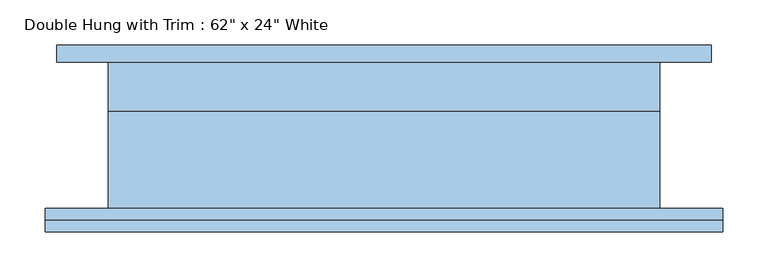
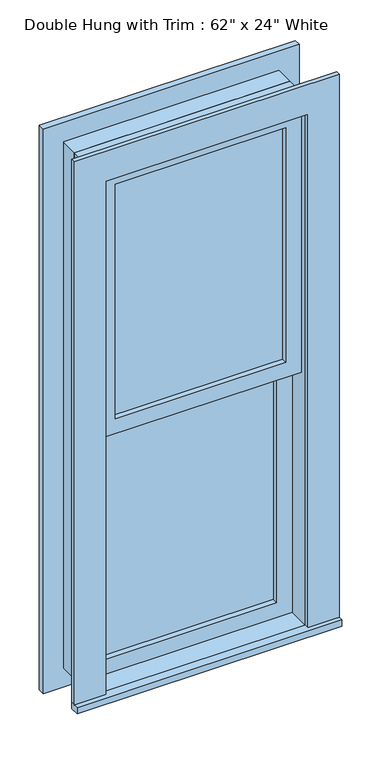
"""IFC4 building model written with IfcOpenShell, lengths in millimetres: window geometry."""

from ifc_helpers import new_model, si_unit, frame, origin, place, context, project, spatial, polyline, outline, extrude, source, transform, mapped, element, save


def window_2795b850(model_context):
    return source(origin(), model_context, "Body", "SweptSolid", [
        extrude(outline(polyline([(-241.3, -1.5875), (-241.3, 11.1125), (241.3, 11.1125), (241.3, -1.5875), (-241.3, -1.5875)])), frame((0.0, 0.0, 977.9), z_axis=(0.0, 0.0, 1.0), x_axis=(1.0, 0.0, 0.0)), (0.0, 0.0, 1.0), 701.675),
        extrude(outline(polyline([(1724.025, -285.75), (933.45, -285.75), (933.45, 285.75), (1724.025, 285.75), (1724.025, -285.75)]), holes=[polyline([(1679.575, -241.3), (1679.575, 241.3), (977.9, 241.3), (977.9, -241.3), (1679.575, -241.3)])]), frame((0.0, -17.4625, 0.0), z_axis=(0.0, 1.0, 0.0), x_axis=(0.0, 0.0, 1.0)), (0.0, 0.0, 1.0), 44.45),
        extrude(outline(polyline([(-374.65, -106.3625), (-374.65, -80.9625), (374.65, -80.9625), (374.65, -106.3625), (-374.65, -106.3625)])), frame((0.0, 0.0, 914.4), z_axis=(0.0, 0.0, 1.0), x_axis=(1.0, 0.0, 0.0)), (0.0, 0.0, 1.0), 19.05),
        extrude(outline(polyline([(2470.15, -285.75), (2470.15, 285.75), (933.45, 285.75), (933.45, 374.65), (2559.05, 374.65), (2559.05, -374.65), (933.45, -374.65), (933.45, -285.75), (2470.15, -285.75)])), frame((0.0, -93.6625, 0.0), z_axis=(0.0, 1.0, 0.0), x_axis=(0.0, 0.0, 1.0)), (0.0, 0.0, 1.0), 12.7),
        extrude(outline(polyline([(2546.35, 361.95), (2546.35, -361.95), (857.25, -361.95), (857.25, 361.95), (2546.35, 361.95)]), holes=[polyline([(2457.45, 273.05), (946.15, 273.05), (946.15, -273.05), (2457.45, -273.05), (2457.45, 273.05)])]), frame((0.0, 80.9625, 0.0), z_axis=(0.0, 1.0, 0.0), x_axis=(0.0, 0.0, 1.0)), (0.0, 0.0, 1.0), 19.05),
        extrude(outline(polyline([(241.3, -33.3375), (241.3, -46.0375), (-241.3, -46.0375), (-241.3, -33.3375), (241.3, -33.3375)])), frame((0.0, 0.0, 1724.025), z_axis=(0.0, 0.0, 1.0), x_axis=(1.0, 0.0, 0.0)), (0.0, 0.0, 1.0), 701.675),
        extrude(outline(polyline([(2470.15, -285.75), (1679.575, -285.75), (1679.575, 285.75), (2470.15, 285.75), (2470.15, -285.75)]), holes=[polyline([(2425.7, -241.3), (2425.7, 241.3), (1724.025, 241.3), (1724.025, -241.3), (2425.7, -241.3)])]), frame((0.0, -61.9125, 0.0), z_axis=(0.0, 1.0, 0.0), x_axis=(0.0, 0.0, 1.0)), (0.0, 0.0, 1.0), 44.45),
        extrude(outline(polyline([(2489.2, -304.8), (914.4, -304.8), (914.4, 304.8), (2489.2, 304.8), (2489.2, -304.8)]), holes=[polyline([(2457.45, -273.05), (2457.45, 273.05), (946.15, 273.05), (946.15, -273.05), (2457.45, -273.05)])]), frame((0.0, 26.9875, 0.0), z_axis=(0.0, 1.0, 0.0), x_axis=(0.0, 0.0, 1.0)), (0.0, 0.0, 1.0), 53.975),
        extrude(outline(polyline([(2489.2, 304.8), (2489.2, -304.8), (914.4, -304.8), (914.4, 304.8), (2489.2, 304.8)]), holes=[polyline([(2470.15, 285.75), (933.45, 285.75), (933.45, -285.75), (2470.15, -285.75), (2470.15, 285.75)])]), frame((0.0, -80.9625, 0.0), z_axis=(0.0, 1.0, 0.0), x_axis=(0.0, 0.0, 1.0)), (0.0, 0.0, 1.0), 107.95),
    ])


if __name__ == "__main__":
    model = new_model("IFC4")
    model_context = context("Model", 3, world=origin())
    ifc_project = project(units=[si_unit("LENGTHUNIT", "METRE", prefix="MILLI")], contexts=[model_context])
    site = spatial("IfcSite", under=ifc_project)
    building = spatial("IfcBuilding", under=site)
    placement = place(None, origin())
    window_shape = window_2795b850(model_context)
    element("IfcWindow", 1, ObjectType="Double Hung with Trim : 62\" x 24\" White", at=placement, inside=building, context=model_context, shape_type="MappedRepresentation", body=[
        mapped(window_shape, transform((0.0, 0.0, 0.0), x_axis=(1.0, 0.0, 0.0), y_axis=(0.0, 1.0, 0.0), z_axis=(0.0, 0.0, 1.0))),
    ])
    save(model, "model.ifc")

# Revit data of these elements
# Type "Double Hung with Trim : 62\" x 24\" White"
#   Type Mark = "77"
#   Construction Type Id = "GSP4R"
#   Assembly Code = "B2020100"
#   Analytic Construction = "1/8 in Pilkington single glazing"
#   Visual Light Transmittance = 0.9
#   Solar Heat Gain Coefficient = 0.78
#   Heat Transfer Coefficient (U) = 3.6886 W/(m²·K)
#   Height = 5' - 2"
#   Default Sill Height = 3' - 0"
#   Trim Projection - Ext. = 0' - 0 1/2"
#   Trim Projection - Int. = 0' - 0 3/4"
#   Trim Width - Exterior = 0' - 3 1/2"
#   Trim Width - Interior = 0' - 3 1/2"
#   Width = 2' - 0"
#   Window Inset = 0' - 0 3/4"
#   COBie.Type = no
#   Glass Pane Material = Glass
#   Sash Material = Sash - White
#   Trim Exterior Material = Trim - White
#   Trim Interior Material = Trim - White
#   Wall Closure = (empty or 0)
# Element 1 (IfcWindow, "Double Hung with Trim : 62\" x 24\" White")
#   Materials on its faces: "Sash - White", "Trim - White", "Glass"
# Materials
#   "Glass": class "Glass", colour RGB 0 128 192, transparency 0.75, Description = "Soda Lime Glass", Cost = 0
#   "Sash - White": class "Wood", colour RGB 255 255 255, transparency 0, Cost = 0
#   "Trim - White": class "Wood", colour RGB 255 255 255, transparency 0, Cost = 0
